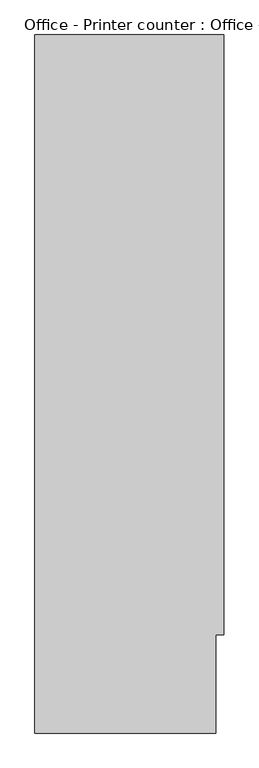
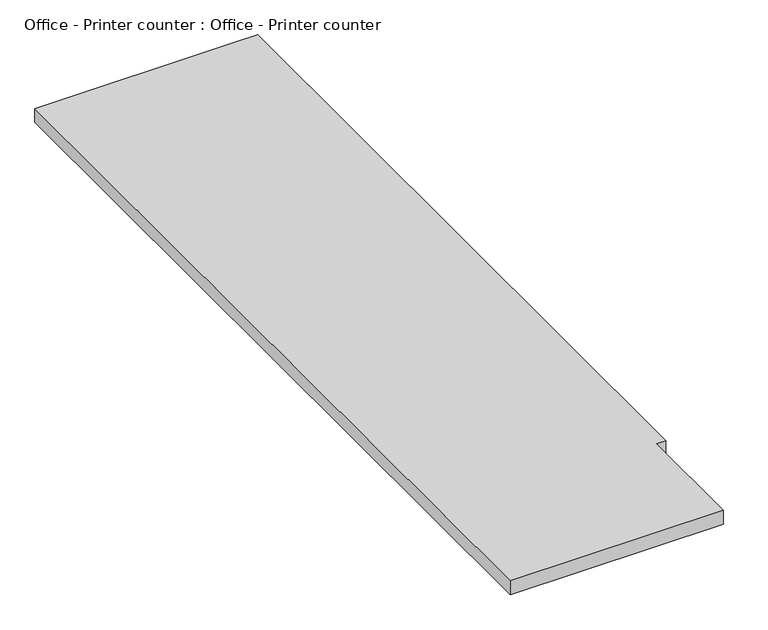
"""IFC4 building model written with IfcOpenShell, lengths in millimetres: furniture geometry, Office - Printer counter : Office - Printer counter."""

import ifcopenshell
import ifcopenshell.guid

model = None  # the IFC model being written
_history = None  # IfcOwnerHistory: only IFC2X3 demands one
_inside = {}  # id of a spatial element -> (the spatial element, [elements in it])
_under = {}  # id of a project, library or spatial element -> (it, [spatial elements below it])
_declared = {}  # id of a project -> (the project, [libraries it declares])
_typed = {}  # id of a type object -> (the type object, [elements of that type])
_made_of = {}  # id of a material, layer set ... -> (it, [elements and type objects made of it])


def new_model(schema):
    """Start an empty IFC model of exactly this schema.

    Asked for "IFC4X3", IfcOpenShell would pick the latest addendum, in which some entities
    have other attributes; the version numbers below select the first issue.
    IFC2X3 requires an IfcOwnerHistory on every rooted entity: one is made here for all.
    """
    global model, _history
    if schema == "IFC4X3":
        model = ifcopenshell.file(schema_version=(4, 3, 0, 0))
    else:
        model = ifcopenshell.file(schema=schema)
    _inside.clear()
    _under.clear()
    _declared.clear()
    _typed.clear()
    _made_of.clear()
    _history = None
    if model.schema == "IFC2X3":
        org = make("IfcOrganization", Name="unknown")
        user = make(
            "IfcPersonAndOrganization",
            ThePerson=make("IfcPerson", FamilyName="unknown"),
            TheOrganization=org,
        )
        app = make(
            "IfcApplication",
            ApplicationDeveloper=org,
            Version="unknown",
            ApplicationFullName="unknown",
            ApplicationIdentifier="unknown",
        )
        _history = make(
            "IfcOwnerHistory",
            OwningUser=user,
            OwningApplication=app,
            ChangeAction="ADDED",
            CreationDate=0,
        )
    return model


def make(cls, **values):
    """One entity of the class cls with the attributes given. An attribute that is None is left unset."""
    return model.create_entity(
        cls, **{name: value for name, value in values.items() if value is not None}
    )


def rooted(cls, **values):
    """An entity with a GlobalId (a new one), such as an element, a storey or a relation."""
    return make(cls, GlobalId=ifcopenshell.guid.new(), OwnerHistory=_history, **values)


def si_unit(unit_type, name, prefix=None):
    """IfcSIUnit, for example si_unit("LENGTHUNIT", "METRE", prefix="MILLI")."""
    return make("IfcSIUnit", UnitType=unit_type, Prefix=prefix, Name=name)


def assignment(units):
    """IfcUnitAssignment: the units of a project."""
    return None if units is None else make("IfcUnitAssignment", Units=units)


def point(xyz):
    """IfcCartesianPoint."""
    return None if xyz is None else make("IfcCartesianPoint", Coordinates=xyz)


def direction(xyz):
    """IfcDirection."""
    return None if xyz is None else make("IfcDirection", DirectionRatios=xyz)


def frame(location, z_axis=None, x_axis=None):
    """IfcAxis2Placement3D, a coordinate frame: its origin and axes. An axis left out is left unset."""
    return make(
        "IfcAxis2Placement3D",
        Location=point(location),
        Axis=direction(z_axis),
        RefDirection=direction(x_axis),
    )


def origin():
    """The frame at (0, 0, 0) with its axes left unset."""
    return frame((0.0, 0.0, 0.0))


def place(relative_to, where):
    """IfcLocalPlacement: puts the frame where relative to a parent placement (None: the world)."""
    return make(
        "IfcLocalPlacement", PlacementRelTo=relative_to, RelativePlacement=where
    )


def context(
    kind, dimensions, precision=None, world=None, true_north=None, identifier=None
):
    """IfcGeometricRepresentationContext, for example the 3D "Model" context."""
    return make(
        "IfcGeometricRepresentationContext",
        ContextIdentifier=identifier,
        ContextType=kind,
        CoordinateSpaceDimension=dimensions,
        Precision=precision,
        WorldCoordinateSystem=world,
        TrueNorth=true_north,
    )


def project(units=None, contexts=None):
    """IfcProject with its units and contexts."""
    return rooted(
        "IfcProject",
        Name="project",
        RepresentationContexts=contexts,
        UnitsInContext=assignment(units),
    )


def spatial(cls, under=None, at=None, **own):
    """A site, building, storey or space (cls), placed at a placement, below another one or the project."""
    s = rooted(cls, ObjectPlacement=at, **own)
    if under is not None:
        _under.setdefault(under.id(), (under, []))[1].append(s)
    return s


def polyline(points):
    """IfcPolyline through the points."""
    return make("IfcPolyline", Points=[point(p) for p in points])


def outline(outer, holes=None, kind="AREA"):
    """IfcArbitraryClosedProfileDef: a profile drawn as a closed curve; with holes, ...WithVoids."""
    if holes is None:
        return make("IfcArbitraryClosedProfileDef", ProfileType=kind, OuterCurve=outer)
    return make(
        "IfcArbitraryProfileDefWithVoids",
        ProfileType=kind,
        OuterCurve=outer,
        InnerCurves=holes,
    )


def extrude(swept, where, along, depth):
    """IfcExtrudedAreaSolid: the profile swept, set in the frame where, extruded along a direction by depth."""
    return make(
        "IfcExtrudedAreaSolid",
        SweptArea=swept,
        Position=where,
        ExtrudedDirection=direction(along),
        Depth=depth,
    )


def shape(context_of_items, identifier, shape_type, items):
    """IfcShapeRepresentation: the items that make up one representation, for example the "Body"."""
    return make(
        "IfcShapeRepresentation",
        ContextOfItems=context_of_items,
        RepresentationIdentifier=identifier,
        RepresentationType=shape_type,
        Items=items,
    )


def source(mapping_origin, context_of_items, identifier, shape_type, items):
    """IfcRepresentationMap: a shape defined once, which mapped items show again and again."""
    return make(
        "IfcRepresentationMap",
        MappingOrigin=mapping_origin,
        MappedRepresentation=shape(context_of_items, identifier, shape_type, items),
    )


def transform(
    local_origin,
    x_axis=None,
    y_axis=None,
    z_axis=None,
    scale=None,
    scale2=None,
    scale3=None,
    uniform=True,
):
    """IfcCartesianTransformationOperator3D, or its non-uniform kind. x_axis, y_axis, z_axis: its Axis1, 2, 3."""
    if uniform:
        return make(
            "IfcCartesianTransformationOperator3D",
            Axis1=direction(x_axis),
            Axis2=direction(y_axis),
            LocalOrigin=point(local_origin),
            Scale=scale,
            Axis3=direction(z_axis),
        )
    return make(
        "IfcCartesianTransformationOperator3DnonUniform",
        Axis1=direction(x_axis),
        Axis2=direction(y_axis),
        LocalOrigin=point(local_origin),
        Scale=scale,
        Axis3=direction(z_axis),
        Scale2=scale2,
        Scale3=scale3,
    )


def mapped(mapping_source, mapping_target):
    """IfcMappedItem: shows the shape of a source again, moved by a transform."""
    return make(
        "IfcMappedItem", MappingSource=mapping_source, MappingTarget=mapping_target
    )


def made_of(thing, what):
    """Note that an element or type object is made of a material, layer set ...; save() writes the relation."""
    if what is not None:
        _made_of.setdefault(what.id(), (what, []))[1].append(thing)
    return thing


def element(
    cls,
    number,
    at=None,
    inside=None,
    cuts=None,
    type_object=None,
    material=None,
    context=None,
    identifier="Body",
    shape_type=None,
    held_by="IfcProductDefinitionShape",
    body=None,
    shapes=None,
    **own,
):
    """One element of the class cls, such as IfcWall. Its Tag is "e" and its number.

    at: its placement. inside: the storey or other place that contains it. cuts: it is an
    opening in that element (IfcRelVoidsElement). A single representation is given by context,
    identifier, shape_type and body (its items); several are given by shapes. held_by: the class
    of the entity that holds the representations. save() writes the other relations.
    """
    e = rooted(cls, Tag="e%d" % number, ObjectPlacement=at, **own)
    if body is not None:
        shapes = [shape(context, identifier, shape_type, body)]
    if shapes is not None:
        e.Representation = make(held_by, Representations=shapes)
    if inside is not None:
        _inside.setdefault(inside.id(), (inside, []))[1].append(e)
    if cuts is not None:
        rooted(
            "IfcRelVoidsElement", RelatingBuildingElement=cuts, RelatedOpeningElement=e
        )
    if type_object is not None:
        _typed.setdefault(type_object.id(), (type_object, []))[1].append(e)
    return made_of(e, material)


def aggregate(whole, parts):
    """IfcRelAggregates: a whole, such as a stair, and the parts it consists of."""
    return rooted("IfcRelAggregates", RelatingObject=whole, RelatedObjects=parts)


def save(model, path):
    """Write the relations noted so far, then the file.

    IfcRelAggregates (storeys below a building ...), IfcRelContainedInSpatialStructure (elements
    in a storey), IfcRelDefinesByType, IfcRelAssociatesMaterial and IfcRelDeclares: one each for
    every whole, place, type object, material and project.
    """
    for whole, parts in _under.values():
        aggregate(whole, parts)
    for where, things in _inside.values():
        rooted(
            "IfcRelContainedInSpatialStructure",
            RelatedElements=things,
            RelatingStructure=where,
        )
    for kind, things in _typed.values():
        rooted("IfcRelDefinesByType", RelatedObjects=things, RelatingType=kind)
    for what, things in _made_of.values():
        rooted("IfcRelAssociatesMaterial", RelatedObjects=things, RelatingMaterial=what)
    for by, libraries in _declared.values():
        rooted("IfcRelDeclares", RelatingContext=by, RelatedDefinitions=libraries)
    model.write(path)


def office_printer_counter_office_printer_counter_b480724c(model_context):
    return source(origin(), model_context, "Body", "SweptSolid", [
        extrude(outline(polyline([(-5456.2375, 15570.2), (-5456.2375, 13716.0), (-5481.6375, 13716.0), (-5481.6375, 13411.2), (-6040.4375, 13411.2), (-6040.4375, 15570.2), (-5512.1175, 15570.2), (-5456.2375, 15570.2)])), frame((0.0, 0.0, 723.9), z_axis=(0.0, 0.0, 1.0), x_axis=(1.0, 0.0, 0.0)), (0.0, 0.0, 1.0), 38.1),
    ])


if __name__ == "__main__":
    model = new_model("IFC4")
    model_context = context("Model", 3, world=origin())
    ifc_project = project(units=[si_unit("LENGTHUNIT", "METRE", prefix="MILLI")], contexts=[model_context])
    site = spatial("IfcSite", under=ifc_project)
    building = spatial("IfcBuilding", under=site)
    placement = place(None, origin())
    office_printer_counter_office_printer_counter_shape = office_printer_counter_office_printer_counter_b480724c(model_context)
    element("IfcFurniture", 1, ObjectType="Office - Printer counter : Office - Printer counter", at=placement, inside=building, context=model_context, shape_type="MappedRepresentation", body=[
        mapped(office_printer_counter_office_printer_counter_shape, transform((0.0, 0.0, 0.0), x_axis=(1.0, 0.0, 0.0), y_axis=(0.0, 1.0, 0.0), z_axis=(0.0, 0.0, 1.0))),
    ])
    save(model, "model.ifc")

# Revit data of these elements
# Type "Office - Printer counter : Office - Printer counter"
#   COBie.Type = no
# Element 1 (IfcFurniture, "Office - Printer counter : Office - Printer counter")
#   Materials on its faces: "Green Laminate"
# Materials
#   "Green Laminate": class "Generic", colour RGB 57 96 54, transparency 0, Cost = 0
